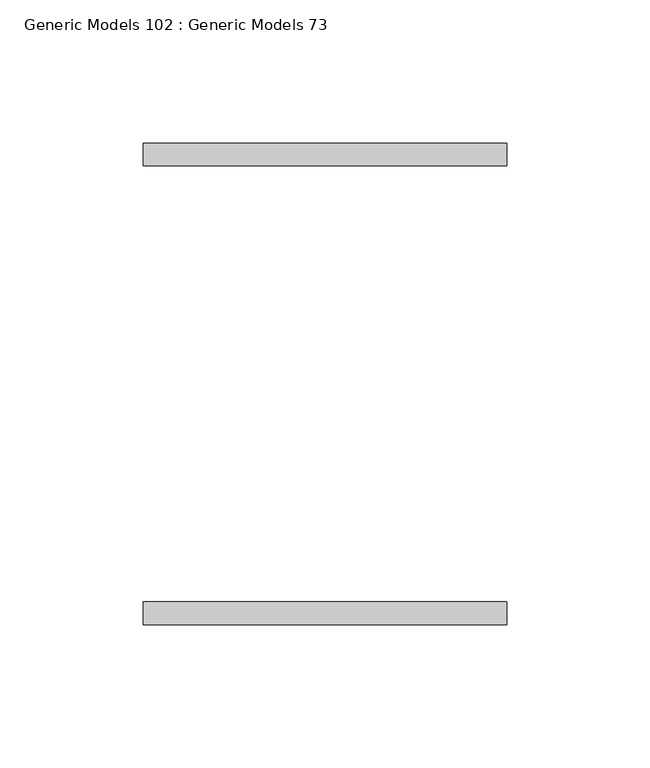
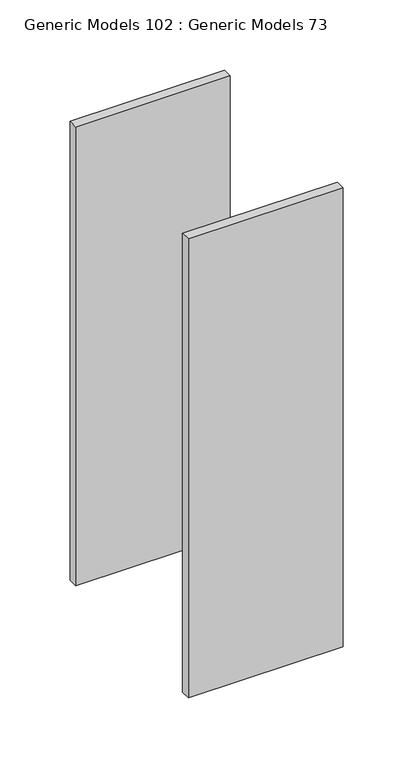
"""IFC4 building model written with IfcOpenShell, lengths in millimetres: proxy geometry, Generic Models 102 : Generic Models 73."""

from ifc_helpers import new_model, si_unit, frame, origin, place, context, project, spatial, polyline, outline, extrude, source, transform, mapped, element, save


def generic_models_102_generic_models_73_db00c337(model_context):
    return source(origin(), model_context, "Body", "SweptSolid", [
        extrude(outline(polyline([(32053.2090778, 30858.4781612), (32053.2090778, 30850.5406612), (31926.2090778, 30850.5406612), (31926.2090778, 30858.4781612), (32053.2090778, 30858.4781612)])), frame((0.0, 0.0, 269146.3375), z_axis=(0.0, 0.0, 1.0), x_axis=(1.0, 0.0, 0.0)), (0.0, 0.0, 1.0), 398.4625),
        extrude(outline(polyline([(32053.2090778, 30698.1406612), (32053.2090778, 30690.2031612), (31926.2090778, 30690.2031612), (31926.2090778, 30698.1406612), (32053.2090778, 30698.1406612)])), frame((0.0, 0.0, 269146.3375), z_axis=(0.0, 0.0, 1.0), x_axis=(1.0, 0.0, 0.0)), (0.0, 0.0, 1.0), 398.4625),
    ])


if __name__ == "__main__":
    model = new_model("IFC4")
    model_context = context("Model", 3, world=origin())
    ifc_project = project(units=[si_unit("LENGTHUNIT", "METRE", prefix="MILLI")], contexts=[model_context])
    site = spatial("IfcSite", under=ifc_project)
    building = spatial("IfcBuilding", under=site)
    placement = place(None, origin())
    generic_models_102_generic_models_73_shape = generic_models_102_generic_models_73_db00c337(model_context)
    element("IfcBuildingElementProxy", 1, Name="Generic Models 102 : Generic Models 73", ObjectType="Generic Models 102 : Generic Models 73", at=placement, inside=building, context=model_context, shape_type="MappedRepresentation", body=[
        mapped(generic_models_102_generic_models_73_shape, transform((0.0, 0.0, 0.0), x_axis=(1.0, 0.0, 0.0), y_axis=(0.0, 1.0, 0.0), z_axis=(0.0, 0.0, 1.0))),
    ])
    save(model, "model.ifc")

# Revit data of these elements
# Element 1 (IfcBuildingElementProxy, "Generic Models 102 : Generic Models 73")
#   Materials on its faces: "5/16 THICK GALV. SADDLE"
# Materials
#   "5/16 THICK GALV. SADDLE": class "Metal", colour RGB 199 199 199, transparency 0, Description = "Carbon steel", Cost = 0
